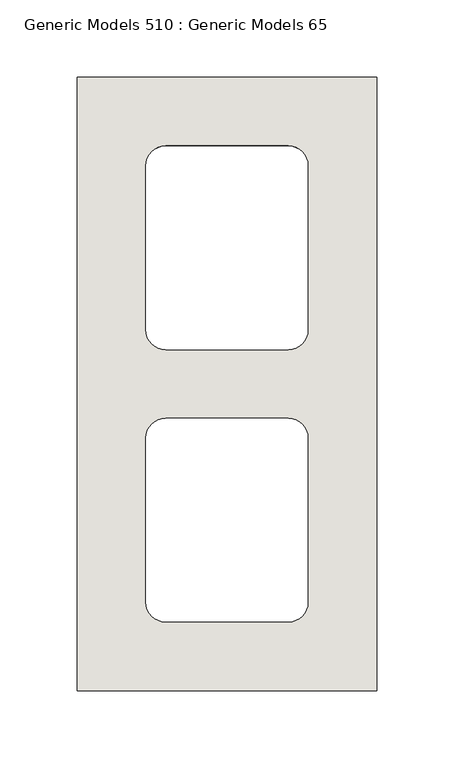
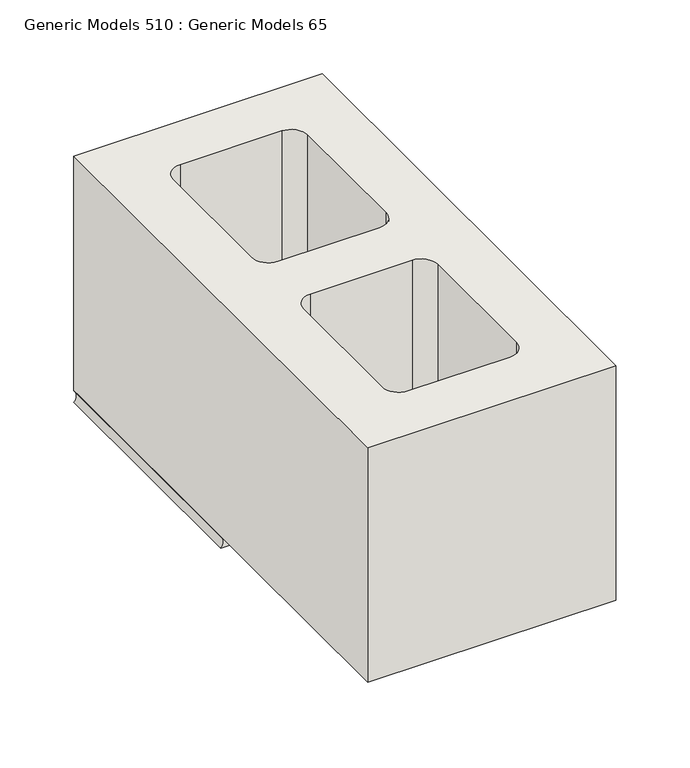
"""IFC4 building model written with IfcOpenShell, lengths in millimetres: wall geometry, Generic Models 510 : Generic Models 65."""

from ifc_helpers import new_model, si_unit, point, frame, frame_2d, origin, place, context, project, spatial, polyline, circle_curve, trimmed, segment, composite_curve, outline, extrude, source, transform, mapped, element, save
from ifc_brep_helpers import plane_surface, revolved_surface, advanced_brep


def generic_models_510_generic_models_65_b7197348(model_context):
    return source(origin(), model_context, "Body", "SolidModel", [
        advanced_brep(
        [(428979.0125, 503.2375, 1025.525), (428785.3375, 503.2375, 1025.525), (428785.3375, 503.2375, 1016.0), (428979.0125, 503.2375, 1016.0), (428979.0125, 701.675, 1025.525), (428979.0125, 701.675, 1016.0), (428785.3375, 701.675, 1016.0), (428785.3375, 701.675, 1025.525), (428934.5625, 538.1625, 1025.525), (428921.8625, 525.4625, 1025.525), (428842.4875, 525.4625, 1025.525), (428829.7875, 538.1625, 1025.525), (428829.7875, 644.525, 1025.525), (428842.4875, 657.225, 1025.525), (428921.8625, 657.225, 1025.525), (428934.5625, 644.525, 1025.525), (428921.8625, 525.4625, 1016.0), (428934.5625, 538.1625, 1016.0), (428842.4875, 525.4625, 1016.0), (428829.7875, 538.1625, 1016.0), (428829.7875, 644.525, 1016.0), (428842.4875, 657.225, 1016.0), (428921.8625, 657.225, 1016.0), (428934.5625, 644.525, 1016.0)],
        [
            (0, 1),
            (1, 2, circle_curve(frame((428780.4545028, 503.2375, 1020.7625), z_axis=(0.0, 1.0, 0.0), x_axis=(1.0, 0.0, 0.0)), 6.8209287)),
            (2, 3),
            (3, 0, circle_curve(frame((428983.8954972, 503.2375, 1020.7625), z_axis=(0.0, 1.0, 0.0), x_axis=(-1.0, 0.0, 0.0)), 6.8209287)),
            (4, 5, circle_curve(frame((428983.8954972, 701.675, 1020.7625), z_axis=(0.0, -1.0, 0.0), x_axis=(-1.0, 0.0, 0.0)), 6.8209287)),
            (5, 6),
            (6, 7, circle_curve(frame((428780.4545028, 701.675, 1020.7625), z_axis=(0.0, -1.0, 0.0), x_axis=(1.0, 0.0, 0.0)), 6.8209287)),
            (7, 4),
            (0, 4),
            (7, 1),
            (8, 9, circle_curve(frame((428921.8625, 538.1625, 1025.525), z_axis=(0.0, 0.0, -1.0), x_axis=(-1.0, 0.0, 0.0)), 12.7)),
            (9, 10),
            (10, 11, circle_curve(frame((428842.4875, 538.1625, 1025.525), z_axis=(0.0, 0.0, -1.0), x_axis=(-1.0, 0.0, 0.0)), 12.7)),
            (11, 12),
            (12, 13, circle_curve(frame((428842.4875, 644.525, 1025.525), z_axis=(0.0, 0.0, -1.0), x_axis=(-1.0, 0.0, 0.0)), 12.7)),
            (13, 14),
            (14, 15, circle_curve(frame((428921.8625, 644.525, 1025.525), z_axis=(0.0, 0.0, -1.0), x_axis=(-1.0, 0.0, 0.0)), 12.7)),
            (15, 8),
            (16, 9),
            (8, 17),
            (17, 16, circle_curve(frame((428921.8625, 538.1625, 1016.0), z_axis=(0.0, 0.0, -1.0), x_axis=(-1.0, 0.0, 0.0)), 12.7)),
            (16, 18),
            (18, 10),
            (18, 19, circle_curve(frame((428842.4875, 538.1625, 1016.0), z_axis=(0.0, 0.0, -1.0), x_axis=(-1.0, 0.0, 0.0)), 12.7)),
            (19, 11),
            (19, 20),
            (20, 12),
            (20, 21, circle_curve(frame((428842.4875, 644.525, 1016.0), z_axis=(0.0, 0.0, -1.0), x_axis=(-1.0, 0.0, 0.0)), 12.7)),
            (21, 13),
            (21, 22),
            (22, 14),
            (22, 23, circle_curve(frame((428921.8625, 644.525, 1016.0), z_axis=(0.0, 0.0, -1.0), x_axis=(-1.0, 0.0, 0.0)), 12.7)),
            (23, 15),
            (23, 17),
            (6, 2),
            (5, 3),
        ],
        [
            plane_surface(frame((428882.175, 503.2375, 1025.921875), z_axis=(0.0, -1.0, 0.0), x_axis=(0.0, 0.0, 1.0))),
            plane_surface(frame((428882.175, 701.675, 1025.921875), z_axis=(0.0, 1.0, 0.0), x_axis=(0.0, 0.0, 1.0))),
            plane_surface(frame((428979.0125, 503.2375, 1025.525), z_axis=(0.0, 0.0, 1.0), x_axis=(0.0, 1.0, 0.0))),
            revolved_surface(polyline([(428909.1625, 538.1625, 1025.525), (428909.1625, 538.1625, 1016.0)]), (428921.8625, 538.1625, 1209.675), (0.0, 0.0, 1.0)),
            plane_surface(frame((428842.4875, 525.4625, 1209.675), z_axis=(0.0, 1.0, 0.0), x_axis=(0.0, 0.0, -1.0))),
            revolved_surface(polyline([(428829.7875, 538.1625, 1025.525), (428829.7875, 538.1625, 1016.0)]), (428842.4875, 538.1625, 1209.675), (0.0, 0.0, 1.0)),
            plane_surface(frame((428829.7875, 644.525, 1209.675), z_axis=(1.0, 0.0, 0.0), x_axis=(0.0, 0.0, -1.0))),
            revolved_surface(polyline([(428829.7875, 644.525, 1025.525), (428829.7875, 644.525, 1016.0)]), (428842.4875, 644.525, 1209.675), (0.0, 0.0, 1.0)),
            plane_surface(frame((428921.8625, 657.225, 1209.675), z_axis=(0.0, -1.0, 0.0), x_axis=(0.0, 0.0, -1.0))),
            revolved_surface(polyline([(428909.1625, 644.525, 1025.525), (428909.1625, 644.525, 1016.0)]), (428921.8625, 644.525, 1209.675), (0.0, 0.0, 1.0)),
            plane_surface(frame((428934.5625, 538.1625, 1209.675), z_axis=(-1.0, 0.0, 0.0), x_axis=(0.0, 0.0, -1.0))),
            revolved_surface(polyline([(428787.2754315, 701.675, 1020.7625), (428787.2754315, 503.2375, 1020.7625)]), (428780.4545028, 503.2375, 1020.7625), (0.0, 1.0, 0.0)),
            plane_surface(frame((428785.3375, 503.2375, 1016.0), z_axis=(0.0, 0.0, -1.0), x_axis=(0.0, 1.0, 0.0))),
            revolved_surface(polyline([(428977.07456850004, 701.675, 1020.7625), (428977.07456850004, 503.2375, 1020.7625)]), (428983.8954972, 503.2375, 1020.7625), (0.0, 1.0, 0.0)),
        ],
        [
            (0, [[1, 2, 3, 4]]),
            (1, [[5, 6, 7, 8]]),
            (2, [[-1, 9, -8, 10], [11, 12, 13, 14, 15, 16, 17, 18]]),
            (3, [[19, -11, 20, 21]]),
            (4, [[-19, 22, 23, -12]]),
            (5, [[-23, 24, 25, -13]]),
            (6, [[-25, 26, 27, -14]]),
            (7, [[-27, 28, 29, -15]]),
            (8, [[-29, 30, 31, -16]]),
            (9, [[-31, 32, 33, -17]]),
            (10, [[-33, 34, -20, -18]]),
            (11, [[-2, -10, -7, 35]]),
            (12, [[-3, -35, -6, 36], [-21, -34, -32, -30, -28, -26, -24, -22]]),
            (13, [[-4, -36, -5, -9]]),
        ],
    ),
        extrude(outline(polyline([(428979.0125, 304.8), (428785.3375, 304.8), (428785.3375, 701.675), (428979.0125, 701.675), (428979.0125, 304.8)]), holes=[composite_curve([segment(polyline([(428934.5625, 538.1625), (428934.5625, 644.525)]), True, "CONTINUOUS"), segment(trimmed(circle_curve(frame_2d((428921.8625, 644.525)), 12.7), [point((428934.5625, 644.525))], [point((428921.8625, 657.225))], True, "CARTESIAN"), True, "CONTINUOUS"), segment(polyline([(428921.8625, 657.225), (428842.4875, 657.225)]), True, "CONTINUOUS"), segment(trimmed(circle_curve(frame_2d((428842.4875, 644.525)), 12.7), [point((428842.4875, 657.225))], [point((428829.7875, 644.525))], True, "CARTESIAN"), True, "CONTINUOUS"), segment(polyline([(428829.7875, 644.525), (428829.7875, 538.1625)]), True, "CONTINUOUS"), segment(trimmed(circle_curve(frame_2d((428842.4875, 538.1625)), 12.7), [point((428829.7875, 538.1625))], [point((428842.4875, 525.4625))], True, "CARTESIAN"), True, "CONTINUOUS"), segment(polyline([(428842.4875, 525.4625), (428921.8625, 525.4625)]), True, "CONTINUOUS"), segment(trimmed(circle_curve(frame_2d((428921.8625, 538.1625)), 12.7), [point((428921.8625, 525.4625))], [point((428934.5625, 538.1625))], True, "CARTESIAN"), True, "CONTINUOUS")], self_intersect=False), composite_curve([segment(polyline([(428829.7875, 468.3125), (428829.7875, 361.95)]), True, "CONTINUOUS"), segment(trimmed(circle_curve(frame_2d((428842.4875, 361.95)), 12.7), [point((428829.7875, 361.95))], [point((428842.4875, 349.25))], True, "CARTESIAN"), True, "CONTINUOUS"), segment(polyline([(428842.4875, 349.25), (428921.8625, 349.25)]), True, "CONTINUOUS"), segment(trimmed(circle_curve(frame_2d((428921.8625, 361.95)), 12.7), [point((428921.8625, 349.25))], [point((428934.5625, 361.95))], True, "CARTESIAN"), True, "CONTINUOUS"), segment(polyline([(428934.5625, 361.95), (428934.5625, 468.3125)]), True, "CONTINUOUS"), segment(trimmed(circle_curve(frame_2d((428921.8625, 468.3125)), 12.7), [point((428934.5625, 468.3125))], [point((428921.8625, 481.0125))], True, "CARTESIAN"), True, "CONTINUOUS"), segment(polyline([(428921.8625, 481.0125), (428842.4875, 481.0125)]), True, "CONTINUOUS"), segment(trimmed(circle_curve(frame_2d((428842.4875, 468.3125)), 12.7), [point((428842.4875, 481.0125))], [point((428829.7875, 468.3125))], True, "CARTESIAN"), True, "CONTINUOUS")], self_intersect=False)]), frame((0.0, 0.0, 1025.525), z_axis=(0.0, 0.0, 1.0), x_axis=(1.0, 0.0, 0.0)), (0.0, 0.0, 1.0), 193.675),
    ])


if __name__ == "__main__":
    model = new_model("IFC4")
    model_context = context("Model", 3, world=origin())
    ifc_project = project(units=[si_unit("LENGTHUNIT", "METRE", prefix="MILLI")], contexts=[model_context])
    site = spatial("IfcSite", under=ifc_project)
    building = spatial("IfcBuilding", under=site)
    placement = place(None, origin())
    generic_models_510_generic_models_65_shape = generic_models_510_generic_models_65_b7197348(model_context)
    element("IfcWall", 1, ObjectType="Generic Models 510 : Generic Models 65", at=placement, inside=building, context=model_context, shape_type="MappedRepresentation", body=[
        mapped(generic_models_510_generic_models_65_shape, transform((0.0, 0.0, 0.0), x_axis=(1.0, 0.0, 0.0), y_axis=(0.0, 1.0, 0.0), z_axis=(0.0, 0.0, 1.0))),
    ])
    save(model, "model.ifc")

# Revit data of these elements
# Element 1 (IfcWall, "Generic Models 510 : Generic Models 65")
#   Materials on its faces: "CMU (SEE 'WALL TAG' FOR SIZE)", "MORTAR JOINT"
# Materials
#   "CMU (SEE 'WALL TAG' FOR SIZE)": class "Masonry", colour RGB 203 203 199, transparency 0, Description = "Concrete masonry units", Cost = 0
#   "MORTAR JOINT": class "Generic", colour RGB 120 120 120, transparency 0, Cost = 0
